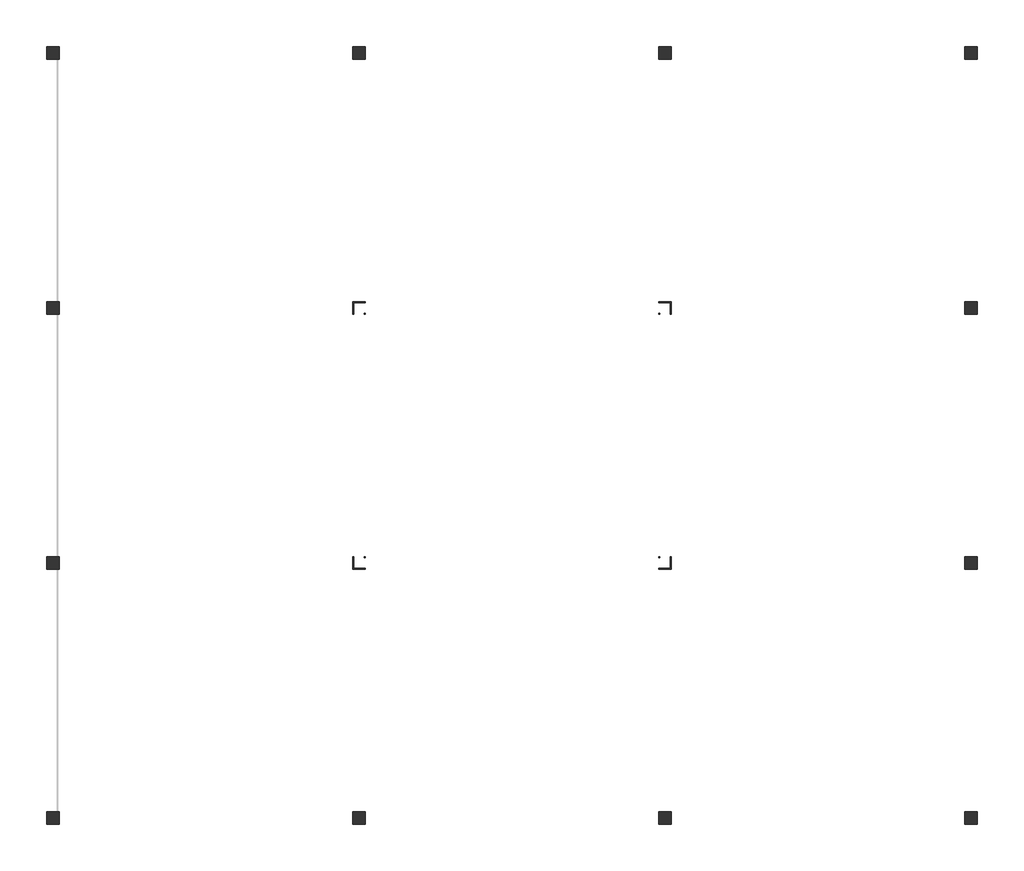
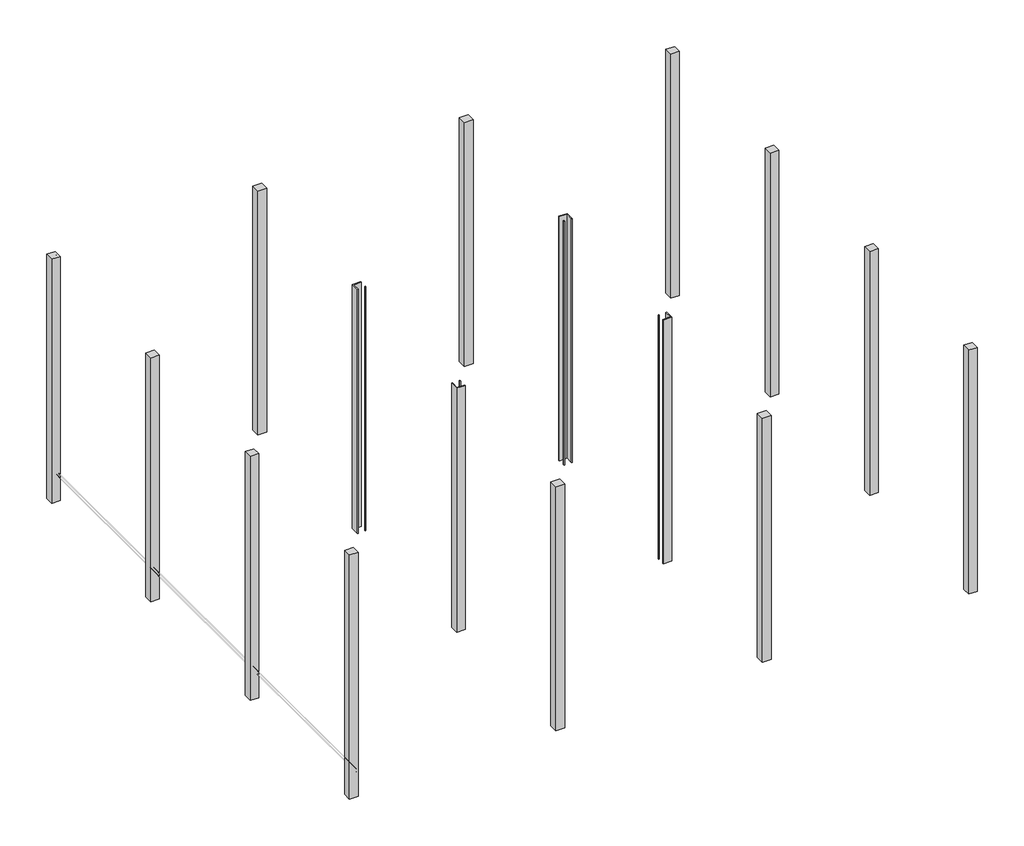
# One storey, part 1 of 2: 16 columns.
"""IFC4 building model written with IfcOpenShell, lengths in millimetres."""

from ifc_helpers import new_model, si_unit, origin, place, context, project, spatial, faceted_brep, element, save

model = new_model("IFC4")

# Units and contexts
model_context = context("Model", 3, world=origin())
ifc_project = project(units=[si_unit("LENGTHUNIT", "METRE", prefix="MILLI")], contexts=[model_context])

# Site, building, storey
site = spatial("IfcSite", under=ifc_project)
building = spatial("IfcBuilding", under=site)
storey = spatial("IfcBuildingStorey", under=building, Name="Foundaiton", Elevation=1000.0)

# Columns
placement = place(None, origin())
element("IfcColumn", 1, ObjectType="Concrete-Rectangular-Column : 250x250 mm", at=placement, inside=storey, context=model_context, shape_type="Brep", body=[
    faceted_brep([(-8833.7181639, -20443.2383613, 8500.0), (-9083.7181639, -20443.2383613, 8500.0), (-9083.7181639, -20693.2383613, 8500.0), (-8833.7181639, -20693.2383613, 8500.0), (-8833.7181639, -20443.2383613, 1000.0), (-8833.7181639, -20693.2383613, 1000.0), (-9083.7181639, -20693.2383613, 1000.0), (-9083.7181639, -20443.2383613, 1000.0), (-8833.7181639, -20443.2383613, 8350.0), (-8833.7181639, -20443.2383613, 8200.0), (-9083.7181639, -20443.2383613, 8200.0), (-9083.7181639, -20443.2383613, 8350.0), (-8833.7181639, -20693.2383613, 8200.0), (-8833.7181639, -20693.2383613, 8350.0)], [[[0, 1, 2, 3]], [[4, 5, 6, 7]], [[1, 0, 8, 9, 4, 7, 10, 11]], [[2, 1, 11, 10, 7, 6]], [[3, 2, 6, 5, 12, 13]], [[0, 3, 13, 12, 5, 4, 9, 8]]]),
])
element("IfcColumn", 2, ObjectType="Concrete-Rectangular-Column : 250x250 mm", at=placement, inside=storey, context=model_context, shape_type="Brep", body=[
    faceted_brep([(-8833.7181639, -15443.2383613, 8500.0), (-9083.7181639, -15443.2383613, 8500.0), (-9083.7181639, -15693.2383613, 8500.0), (-8833.7181639, -15693.2383613, 8500.0), (-8833.7181639, -15443.2383613, 1000.0), (-8833.7181639, -15693.2383613, 1000.0), (-9083.7181639, -15693.2383613, 1000.0), (-9083.7181639, -15443.2383613, 1000.0), (-8833.7181639, -15443.2383613, 8350.0), (-8833.7181639, -15443.2383613, 8200.0), (-9083.7181639, -15443.2383613, 8200.0), (-9083.7181639, -15443.2383613, 8350.0), (-9083.7181639, -15693.2383613, 8200.0), (-9083.7181639, -15693.2383613, 8350.0), (-8833.7181639, -15693.2383613, 8200.0), (-8833.7181639, -15693.2383613, 8350.0)], [[[0, 1, 2, 3]], [[4, 5, 6, 7]], [[1, 0, 8, 9, 4, 7, 10, 11]], [[2, 1, 11, 10, 7, 6, 12, 13]], [[3, 2, 13, 12, 6, 5, 14, 15]], [[0, 3, 15, 14, 5, 4, 9, 8]]]),
])
element("IfcColumn", 3, ObjectType="Concrete-Rectangular-Column : 250x250 mm", at=placement, inside=storey, context=model_context, shape_type="Brep", body=[
    faceted_brep([(-8833.7181639, -10443.2383613, 8500.0), (-9083.7181639, -10443.2383613, 8500.0), (-9083.7181639, -10693.2383613, 8500.0), (-8833.7181639, -10693.2383613, 8500.0), (-8833.7181639, -10443.2383613, 1000.0), (-8833.7181639, -10693.2383613, 1000.0), (-9083.7181639, -10693.2383613, 1000.0), (-9083.7181639, -10443.2383613, 1000.0), (-8833.7181639, -10443.2383613, 8350.0), (-8833.7181639, -10443.2383613, 8200.0), (-9083.7181639, -10443.2383613, 8200.0), (-9083.7181639, -10443.2383613, 8350.0), (-9083.7181639, -10693.2383613, 8200.0), (-9083.7181639, -10693.2383613, 8350.0), (-8833.7181639, -10693.2383613, 8200.0), (-8833.7181639, -10693.2383613, 8350.0)], [[[0, 1, 2, 3]], [[4, 5, 6, 7]], [[1, 0, 8, 9, 4, 7, 10, 11]], [[2, 1, 11, 10, 7, 6, 12, 13]], [[3, 2, 13, 12, 6, 5, 14, 15]], [[0, 3, 15, 14, 5, 4, 9, 8]]]),
])
element("IfcColumn", 4, ObjectType="Concrete-Rectangular-Column : 250x250 mm", at=placement, inside=storey, context=model_context, shape_type="Brep", body=[
    faceted_brep([(-8833.7181639, -5443.2383613, 8500.0), (-9083.7181639, -5443.2383613, 8500.0), (-9083.7181639, -5693.2383613, 8500.0), (-8833.7181639, -5693.2383613, 8500.0), (-8833.7181639, -5443.2383613, 1000.0), (-8833.7181639, -5693.2383613, 1000.0), (-9083.7181639, -5693.2383613, 1000.0), (-9083.7181639, -5443.2383613, 1000.0), (-8833.7181639, -5443.2383613, 8350.0), (-8833.7181639, -5443.2383613, 8200.0), (-9083.7181639, -5693.2383613, 8200.0), (-9083.7181639, -5693.2383613, 8350.0), (-8833.7181639, -5693.2383613, 8200.0), (-8833.7181639, -5693.2383613, 8350.0)], [[[0, 1, 2, 3]], [[4, 5, 6, 7]], [[1, 0, 8, 9, 4, 7]], [[2, 1, 7, 6, 10, 11]], [[3, 2, 11, 10, 6, 5, 12, 13]], [[0, 3, 13, 12, 5, 4, 9, 8]]]),
])
element("IfcColumn", 5, ObjectType="Concrete-Rectangular-Column : 250x250 mm", at=placement, inside=storey, context=model_context, shape_type="Brep", body=[
    faceted_brep([(-2833.7181639, -20443.2383613, 8500.0), (-3083.7181639, -20443.2383613, 8500.0), (-3083.7181639, -20693.2383613, 8500.0), (-2833.7181639, -20693.2383613, 8500.0), (-2833.7181639, -20443.2383613, 1000.0), (-2833.7181639, -20693.2383613, 1000.0), (-3083.7181639, -20693.2383613, 1000.0), (-3083.7181639, -20443.2383613, 1000.0), (-2833.7181639, -20443.2383613, 8350.0), (-2833.7181639, -20443.2383613, 8200.0), (-3083.7181639, -20443.2383613, 8200.0), (-3083.7181639, -20443.2383613, 8350.0), (-3083.7181639, -20693.2383613, 8200.0), (-3083.7181639, -20693.2383613, 8350.0), (-2833.7181639, -20693.2383613, 8200.0), (-2833.7181639, -20693.2383613, 8350.0)], [[[0, 1, 2, 3]], [[4, 5, 6, 7]], [[1, 0, 8, 9, 4, 7, 10, 11]], [[2, 1, 11, 10, 7, 6, 12, 13]], [[3, 2, 13, 12, 6, 5, 14, 15]], [[0, 3, 15, 14, 5, 4, 9, 8]]]),
])
element("IfcColumn", 6, ObjectType="Concrete-Rectangular-Column : 250x250 mm", at=placement, inside=storey, context=model_context, shape_type="Brep", body=[
    faceted_brep([(-2833.7181639, -15468.2383613, 8500.0), (-2833.7181639, -15443.2383613, 8500.0), (-2858.7181639, -15443.2383613, 8500.0), (-2858.7181639, -15468.2383613, 8500.0), (-2833.7181639, -15443.2383613, 1000.0), (-2833.7181639, -15468.2383613, 1000.0), (-2858.7181639, -15468.2383613, 1000.0), (-2858.7181639, -15443.2383613, 1000.0), (-2833.7181639, -15443.2383613, 8350.0), (-2833.7181639, -15443.2383613, 8200.0), (-2858.7181639, -15443.2383613, 8200.0), (-2858.7181639, -15443.2383613, 8350.0), (-2833.7181639, -15468.2383613, 8350.0), (-2833.7181639, -15468.2383613, 8200.0)], [[[0, 1, 2, 3]], [[4, 5, 6, 7]], [[1, 8, 9, 4, 7, 10, 11, 2]], [[4, 9, 8, 1, 0, 12, 13, 5]], [[5, 13, 12, 0, 3, 6]], [[3, 2, 11, 10, 7, 6]]]),
    faceted_brep([(-3083.7181639, -15693.2383613, 8500.0), (-3083.7181639, -15443.2383613, 8500.0), (-3083.7181639, -15443.2383613, 8350.0), (-3083.7181639, -15443.2383613, 8200.0), (-3083.7181639, -15443.2383613, 1000.0), (-3083.7181639, -15693.2383613, 1000.0), (-3083.7181639, -15693.2383613, 8200.0), (-3083.7181639, -15693.2383613, 8350.0), (-2833.7181639, -15693.2383613, 8500.0), (-2833.7181639, -15693.2383613, 1000.0), (-2833.7181639, -15693.2383613, 8200.0), (-2833.7181639, -15693.2383613, 8350.0), (-2833.7181639, -15668.2383613, 1000.0), (-3058.7181639, -15668.2383613, 1000.0), (-3058.7181639, -15668.2383613, 8500.0), (-2833.7181639, -15668.2383613, 8500.0), (-2833.7181639, -15668.2383613, 8350.0), (-2833.7181639, -15668.2383613, 8200.0), (-3058.7181639, -15468.2383613, 1000.0), (-3058.7181639, -15443.2383613, 1000.0), (-3058.7181639, -15443.2383613, 8200.0), (-3058.7181639, -15443.2383613, 8350.0), (-3058.7181639, -15443.2383613, 8500.0)], [[[0, 1, 2, 3, 4, 5, 6, 7]], [[8, 0, 7, 6, 5, 9, 10, 11]], [[12, 13, 14, 15, 16, 17]], [[14, 13, 18, 19, 20, 21, 22]], [[9, 5, 4, 19, 18, 13, 12]], [[8, 11, 10, 9, 12, 17, 16, 15]], [[1, 0, 8, 15, 14, 22]], [[4, 3, 2, 1, 22, 21, 20, 19]]]),
])
element("IfcColumn", 7, ObjectType="Concrete-Rectangular-Column : 250x250 mm", at=placement, inside=storey, context=model_context, shape_type="Brep", body=[
    faceted_brep([(-2833.7181639, -10443.2383613, 8500.0), (-3083.7181639, -10443.2383613, 8500.0), (-3083.7181639, -10693.2383613, 8500.0), (-3058.7181639, -10693.2383613, 8500.0), (-3058.7181639, -10468.2383613, 8500.0), (-2833.7181639, -10468.2383613, 8500.0), (-3083.7181639, -10693.2383613, 1000.0), (-3083.7181639, -10443.2383613, 1000.0), (-2833.7181639, -10443.2383613, 1000.0), (-2833.7181639, -10468.2383613, 1000.0), (-3058.7181639, -10468.2383613, 1000.0), (-3058.7181639, -10668.2383613, 1000.0), (-3058.7181639, -10693.2383613, 1000.0), (-2833.7181639, -10443.2383613, 8350.0), (-2833.7181639, -10443.2383613, 8200.0), (-3083.7181639, -10443.2383613, 8200.0), (-3083.7181639, -10443.2383613, 8350.0), (-3083.7181639, -10693.2383613, 8200.0), (-3083.7181639, -10693.2383613, 8350.0), (-3058.7181639, -10693.2383613, 8200.0), (-3058.7181639, -10693.2383613, 8350.0), (-2833.7181639, -10468.2383613, 8350.0), (-2833.7181639, -10468.2383613, 8200.0)], [[[0, 1, 2, 3, 4, 5]], [[6, 7, 8, 9, 10, 11, 12]], [[1, 0, 13, 14, 8, 7, 15, 16]], [[2, 1, 16, 15, 7, 6, 17, 18]], [[2, 18, 17, 6, 12, 19, 20, 3]], [[8, 14, 13, 0, 5, 21, 22, 9]], [[10, 9, 22, 21, 5, 4]], [[10, 4, 3, 20, 19, 12, 11]]]),
    faceted_brep([(-2833.7181639, -10668.2383613, 8500.0), (-2833.7181639, -10668.2383613, 8350.0), (-2833.7181639, -10668.2383613, 8200.0), (-2833.7181639, -10668.2383613, 1000.0), (-2858.7181639, -10668.2383613, 1000.0), (-2858.7181639, -10668.2383613, 8500.0), (-2858.7181639, -10693.2383613, 8500.0), (-2858.7181639, -10693.2383613, 1000.0), (-2858.7181639, -10693.2383613, 8200.0), (-2858.7181639, -10693.2383613, 8350.0), (-2833.7181639, -10693.2383613, 1000.0), (-2833.7181639, -10693.2383613, 8500.0), (-2833.7181639, -10693.2383613, 8350.0), (-2833.7181639, -10693.2383613, 8200.0)], [[[0, 1, 2, 3, 4, 5]], [[6, 5, 4, 7, 8, 9]], [[3, 10, 7, 4]], [[11, 12, 13, 10, 3, 2, 1, 0]], [[11, 0, 5, 6]], [[10, 13, 12, 11, 6, 9, 8, 7]]]),
])
element("IfcColumn", 8, ObjectType="Concrete-Rectangular-Column : 250x250 mm", at=placement, inside=storey, context=model_context, shape_type="Brep", body=[
    faceted_brep([(-2833.7181639, -5443.2383613, 8500.0), (-3083.7181639, -5443.2383613, 8500.0), (-3083.7181639, -5693.2383613, 8500.0), (-2833.7181639, -5693.2383613, 8500.0), (-2833.7181639, -5443.2383613, 1000.0), (-2833.7181639, -5693.2383613, 1000.0), (-3083.7181639, -5693.2383613, 1000.0), (-3083.7181639, -5443.2383613, 1000.0), (-2833.7181639, -5443.2383613, 8350.0), (-2833.7181639, -5443.2383613, 8200.0), (-3083.7181639, -5443.2383613, 8200.0), (-3083.7181639, -5443.2383613, 8350.0), (-3083.7181639, -5693.2383613, 8200.0), (-3083.7181639, -5693.2383613, 8350.0), (-2833.7181639, -5693.2383613, 8200.0), (-2833.7181639, -5693.2383613, 8350.0)], [[[0, 1, 2, 3]], [[4, 5, 6, 7]], [[1, 0, 8, 9, 4, 7, 10, 11]], [[2, 1, 11, 10, 7, 6, 12, 13]], [[3, 2, 13, 12, 6, 5, 14, 15]], [[0, 3, 15, 14, 5, 4, 9, 8]]]),
])
element("IfcColumn", 9, ObjectType="Concrete-Rectangular-Column : 250x250 mm", at=placement, inside=storey, context=model_context, shape_type="Brep", body=[
    faceted_brep([(3166.2818361, -20443.2383613, 8500.0), (2916.2818361, -20443.2383613, 8500.0), (2916.2818361, -20693.2383613, 8500.0), (3166.2818361, -20693.2383613, 8500.0), (3166.2818361, -20443.2383613, 1000.0), (3166.2818361, -20693.2383613, 1000.0), (2916.2818361, -20693.2383613, 1000.0), (2916.2818361, -20443.2383613, 1000.0), (3166.2818361, -20443.2383613, 8350.0), (3166.2818361, -20443.2383613, 8200.0), (2916.2818361, -20443.2383613, 8200.0), (2916.2818361, -20443.2383613, 8350.0), (2916.2818361, -20693.2383613, 8200.0), (2916.2818361, -20693.2383613, 8350.0), (3166.2818361, -20693.2383613, 8200.0), (3166.2818361, -20693.2383613, 8350.0)], [[[0, 1, 2, 3]], [[4, 5, 6, 7]], [[1, 0, 8, 9, 4, 7, 10, 11]], [[2, 1, 11, 10, 7, 6, 12, 13]], [[3, 2, 13, 12, 6, 5, 14, 15]], [[0, 3, 15, 14, 5, 4, 9, 8]]]),
])
element("IfcColumn", 10, ObjectType="Concrete-Rectangular-Column : 250x250 mm", at=placement, inside=storey, context=model_context, shape_type="Brep", body=[
    faceted_brep([(2916.2818361, -15443.2383613, 8500.0), (2916.2818361, -15468.2383613, 8500.0), (2941.2818361, -15468.2383613, 8500.0), (2941.2818361, -15443.2383613, 8500.0), (2916.2818361, -15468.2383613, 1000.0), (2916.2818361, -15443.2383613, 1000.0), (2941.2818361, -15443.2383613, 1000.0), (2941.2818361, -15468.2383613, 1000.0), (2916.2818361, -15443.2383613, 8350.0), (2916.2818361, -15443.2383613, 8200.0), (2916.2818361, -15468.2383613, 8200.0), (2916.2818361, -15468.2383613, 8350.0), (2941.2818361, -15443.2383613, 8200.0), (2941.2818361, -15443.2383613, 8350.0)], [[[0, 1, 2, 3]], [[4, 5, 6, 7]], [[0, 8, 9, 5, 4, 10, 11, 1]], [[1, 11, 10, 4, 7, 2]], [[3, 2, 7, 6, 12, 13]], [[5, 9, 8, 0, 3, 13, 12, 6]]]),
    faceted_brep([(3166.2818361, -15443.2383613, 8500.0), (3166.2818361, -15443.2383613, 8350.0), (3166.2818361, -15443.2383613, 8200.0), (3166.2818361, -15443.2383613, 1000.0), (3141.2818361, -15443.2383613, 1000.0), (3141.2818361, -15443.2383613, 8200.0), (3141.2818361, -15443.2383613, 8350.0), (3141.2818361, -15443.2383613, 8500.0), (3166.2818361, -15693.2383613, 8500.0), (2916.2818361, -15693.2383613, 8500.0), (2916.2818361, -15693.2383613, 8350.0), (2916.2818361, -15693.2383613, 8200.0), (2916.2818361, -15693.2383613, 1000.0), (3166.2818361, -15693.2383613, 1000.0), (3166.2818361, -15693.2383613, 8200.0), (3166.2818361, -15693.2383613, 8350.0), (3141.2818361, -15668.2383613, 1000.0), (2916.2818361, -15668.2383613, 1000.0), (2916.2818361, -15668.2383613, 8200.0), (2916.2818361, -15668.2383613, 8350.0), (2916.2818361, -15668.2383613, 8500.0), (3141.2818361, -15668.2383613, 8500.0), (3141.2818361, -15468.2383613, 1000.0)], [[[0, 1, 2, 3, 4, 5, 6, 7]], [[8, 9, 10, 11, 12, 13, 14, 15]], [[0, 8, 15, 14, 13, 3, 2, 1]], [[16, 17, 18, 19, 20, 21]], [[16, 21, 7, 6, 5, 4, 22]], [[3, 13, 12, 17, 16, 22, 4]], [[12, 11, 10, 9, 20, 19, 18, 17]], [[9, 8, 0, 7, 21, 20]]]),
])
element("IfcColumn", 11, ObjectType="Concrete-Rectangular-Column : 250x250 mm", at=placement, inside=storey, context=model_context, shape_type="Brep", body=[
    faceted_brep([(3166.2818361, -10443.2383613, 8500.0), (2916.2818361, -10443.2383613, 8500.0), (2916.2818361, -10468.2383613, 8500.0), (3141.2818361, -10468.2383613, 8500.0), (3141.2818361, -10693.2383613, 8500.0), (3166.2818361, -10693.2383613, 8500.0), (3166.2818361, -10443.2383613, 8350.0), (3166.2818361, -10443.2383613, 8200.0), (3166.2818361, -10443.2383613, 1000.0), (2916.2818361, -10443.2383613, 1000.0), (2916.2818361, -10443.2383613, 8200.0), (2916.2818361, -10443.2383613, 8350.0), (2916.2818361, -10468.2383613, 1000.0), (2916.2818361, -10468.2383613, 8200.0), (2916.2818361, -10468.2383613, 8350.0), (3166.2818361, -10693.2383613, 8350.0), (3166.2818361, -10693.2383613, 8200.0), (3166.2818361, -10693.2383613, 1000.0), (3141.2818361, -10468.2383613, 1000.0), (3141.2818361, -10668.2383613, 1000.0), (3141.2818361, -10693.2383613, 1000.0), (3141.2818361, -10693.2383613, 8200.0), (3141.2818361, -10693.2383613, 8350.0)], [[[0, 1, 2, 3, 4, 5]], [[1, 0, 6, 7, 8, 9, 10, 11]], [[1, 11, 10, 9, 12, 13, 14, 2]], [[0, 5, 15, 16, 17, 8, 7, 6]], [[12, 18, 3, 2, 14, 13]], [[3, 18, 19, 20, 21, 22, 4]], [[8, 17, 20, 19, 18, 12, 9]], [[17, 16, 15, 5, 4, 22, 21, 20]]]),
    faceted_brep([(2916.2818361, -10693.2383613, 1000.0), (2916.2818361, -10668.2383613, 1000.0), (2941.2818361, -10668.2383613, 1000.0), (2941.2818361, -10693.2383613, 1000.0), (2916.2818361, -10693.2383613, 8500.0), (2916.2818361, -10693.2383613, 8350.0), (2916.2818361, -10693.2383613, 8200.0), (2941.2818361, -10693.2383613, 8200.0), (2941.2818361, -10693.2383613, 8350.0), (2941.2818361, -10693.2383613, 8500.0), (2916.2818361, -10668.2383613, 8200.0), (2916.2818361, -10668.2383613, 8350.0), (2916.2818361, -10668.2383613, 8500.0), (2941.2818361, -10668.2383613, 8500.0)], [[[0, 1, 2, 3]], [[4, 5, 6, 0, 3, 7, 8, 9]], [[1, 10, 11, 12, 13, 2]], [[13, 9, 8, 7, 3, 2]], [[0, 6, 5, 4, 12, 11, 10, 1]], [[12, 4, 9, 13]]]),
])
element("IfcColumn", 12, ObjectType="Concrete-Rectangular-Column : 250x250 mm", at=placement, inside=storey, context=model_context, shape_type="Brep", body=[
    faceted_brep([(3166.2818361, -5443.2383613, 8500.0), (2916.2818361, -5443.2383613, 8500.0), (2916.2818361, -5693.2383613, 8500.0), (3166.2818361, -5693.2383613, 8500.0), (3166.2818361, -5443.2383613, 1000.0), (3166.2818361, -5693.2383613, 1000.0), (2916.2818361, -5693.2383613, 1000.0), (2916.2818361, -5443.2383613, 1000.0), (3166.2818361, -5443.2383613, 8350.0), (3166.2818361, -5443.2383613, 8200.0), (2916.2818361, -5443.2383613, 8200.0), (2916.2818361, -5443.2383613, 8350.0), (2916.2818361, -5693.2383613, 8200.0), (2916.2818361, -5693.2383613, 8350.0), (3166.2818361, -5693.2383613, 8200.0), (3166.2818361, -5693.2383613, 8350.0)], [[[0, 1, 2, 3]], [[4, 5, 6, 7]], [[1, 0, 8, 9, 4, 7, 10, 11]], [[2, 1, 11, 10, 7, 6, 12, 13]], [[3, 2, 13, 12, 6, 5, 14, 15]], [[0, 3, 15, 14, 5, 4, 9, 8]]]),
])
element("IfcColumn", 13, ObjectType="Concrete-Rectangular-Column : 250x250 mm", at=placement, inside=storey, context=model_context, shape_type="Brep", body=[
    faceted_brep([(9166.2818361, -20443.2383613, 8500.0), (8916.2818361, -20443.2383613, 8500.0), (8916.2818361, -20693.2383613, 8500.0), (9166.2818361, -20693.2383613, 8500.0), (9166.2818361, -20443.2383613, 1000.0), (9166.2818361, -20693.2383613, 1000.0), (8916.2818361, -20693.2383613, 1000.0), (8916.2818361, -20443.2383613, 1000.0), (9166.2818361, -20443.2383613, 8350.0), (9166.2818361, -20443.2383613, 8200.0), (8916.2818361, -20443.2383613, 8200.0), (8916.2818361, -20443.2383613, 8350.0), (8916.2818361, -20693.2383613, 8200.0), (8916.2818361, -20693.2383613, 8350.0)], [[[0, 1, 2, 3]], [[4, 5, 6, 7]], [[1, 0, 8, 9, 4, 7, 10, 11]], [[2, 1, 11, 10, 7, 6, 12, 13]], [[3, 2, 13, 12, 6, 5]], [[0, 3, 5, 4, 9, 8]]]),
])
element("IfcColumn", 14, ObjectType="Concrete-Rectangular-Column : 250x250 mm", at=placement, inside=storey, context=model_context, shape_type="Brep", body=[
    faceted_brep([(9166.2818361, -15443.2383613, 8500.0), (8916.2818361, -15443.2383613, 8500.0), (8916.2818361, -15693.2383613, 8500.0), (9166.2818361, -15693.2383613, 8500.0), (9166.2818361, -15443.2383613, 1000.0), (9166.2818361, -15693.2383613, 1000.0), (8916.2818361, -15693.2383613, 1000.0), (8916.2818361, -15443.2383613, 1000.0), (9166.2818361, -15443.2383613, 8350.0), (9166.2818361, -15443.2383613, 8200.0), (8916.2818361, -15443.2383613, 8200.0), (8916.2818361, -15443.2383613, 8350.0), (8916.2818361, -15693.2383613, 8200.0), (8916.2818361, -15693.2383613, 8350.0), (9166.2818361, -15693.2383613, 8200.0), (9166.2818361, -15693.2383613, 8350.0)], [[[0, 1, 2, 3]], [[4, 5, 6, 7]], [[1, 0, 8, 9, 4, 7, 10, 11]], [[2, 1, 11, 10, 7, 6, 12, 13]], [[3, 2, 13, 12, 6, 5, 14, 15]], [[0, 3, 15, 14, 5, 4, 9, 8]]]),
])
element("IfcColumn", 15, ObjectType="Concrete-Rectangular-Column : 250x250 mm", at=placement, inside=storey, context=model_context, shape_type="Brep", body=[
    faceted_brep([(9166.2818361, -10443.2383613, 8500.0), (8916.2818361, -10443.2383613, 8500.0), (8916.2818361, -10693.2383613, 8500.0), (9166.2818361, -10693.2383613, 8500.0), (9166.2818361, -10443.2383613, 1000.0), (9166.2818361, -10693.2383613, 1000.0), (8916.2818361, -10693.2383613, 1000.0), (8916.2818361, -10443.2383613, 1000.0), (9166.2818361, -10443.2383613, 8350.0), (9166.2818361, -10443.2383613, 8200.0), (8916.2818361, -10443.2383613, 8200.0), (8916.2818361, -10443.2383613, 8350.0), (8916.2818361, -10693.2383613, 8200.0), (8916.2818361, -10693.2383613, 8350.0), (9166.2818361, -10693.2383613, 8200.0), (9166.2818361, -10693.2383613, 8350.0)], [[[0, 1, 2, 3]], [[4, 5, 6, 7]], [[1, 0, 8, 9, 4, 7, 10, 11]], [[2, 1, 11, 10, 7, 6, 12, 13]], [[3, 2, 13, 12, 6, 5, 14, 15]], [[0, 3, 15, 14, 5, 4, 9, 8]]]),
])
element("IfcColumn", 16, ObjectType="Concrete-Rectangular-Column : 250x250 mm", at=placement, inside=storey, context=model_context, shape_type="Brep", body=[
    faceted_brep([(9166.2818361, -5443.2383613, 8500.0), (8916.2818361, -5443.2383613, 8500.0), (8916.2818361, -5693.2383613, 8500.0), (9166.2818361, -5693.2383613, 8500.0), (9166.2818361, -5443.2383613, 1000.0), (9166.2818361, -5693.2383613, 1000.0), (8916.2818361, -5693.2383613, 1000.0), (8916.2818361, -5443.2383613, 1000.0), (8916.2818361, -5443.2383613, 8200.0), (8916.2818361, -5443.2383613, 8350.0), (8916.2818361, -5693.2383613, 8200.0), (8916.2818361, -5693.2383613, 8350.0), (9166.2818361, -5693.2383613, 8200.0), (9166.2818361, -5693.2383613, 8350.0)], [[[0, 1, 2, 3]], [[4, 5, 6, 7]], [[1, 0, 4, 7, 8, 9]], [[2, 1, 9, 8, 7, 6, 10, 11]], [[3, 2, 11, 10, 6, 5, 12, 13]], [[0, 3, 13, 12, 5, 4]]]),
])

save(model, "model.ifc")

# Revit data of these elements
# Project information
#   Project Issue Date = "Issue Date"
#   Project Status = "Project Status"
#   Client Name = "Owner"
#   Project Address = "Enter address here"
#   Project Name = "Project Name"
#   Project Number = "Project Number"
# Grids (mm)
#   "1": line (-8958.718, -21798.806) -> (-8958.718, -2308.142)
#   "2": line (-2958.718, -21798.806) -> (-2958.718, -2308.142)
#   "3": line (3041.282, -21798.806) -> (3041.282, -2308.142)
#   "4": line (9041.282, -21798.806) -> (9041.282, -2308.142)
#   "A": line (12739.772, -20568.238) -> (-12295.272, -20568.238)
#   "B": line (12739.772, -15568.238) -> (-12295.272, -15568.238)
#   "C": line (12739.772, -10568.238) -> (-12295.272, -10568.238)
#   "D": line (12739.772, -5568.238) -> (-12295.272, -5568.238)
# Type "Concrete-Rectangular-Column : 250x250 mm"
#   b = 250 mm
#   h = 250 mm
#   Structural Material [instance default] = Concrete, Cast-in-Place gray
# Elements 1, 2, 3, 5, 6, 7, 9, 10, 11, 13, 14, 15 (IfcColumn, "Concrete-Rectangular-Column : 250x250 mm")
#   Export to IFC = 0
#   Structural Material = Concrete, Cast-in-Place gray
#   Phase Created = New Construction
#   Materials on its faces: "Concrete, Cast-in-Place gray"
# Elements 4, 8, 12, 16 (IfcColumn, "Concrete-Rectangular-Column : 250x250 mm")
#   Structural Material = Concrete, Cast-in-Place gray
#   Phase Created = New Construction
#   Materials on its faces: "Concrete, Cast-in-Place gray"
# Materials
#   "Concrete, Cast-in-Place gray": class "Concrete", colour RGB 192 192 192, transparency 0, Description = "Cast-in-place concrete", Cost = 0
